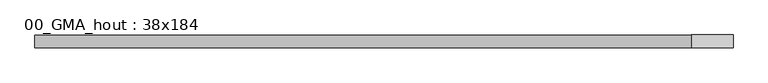
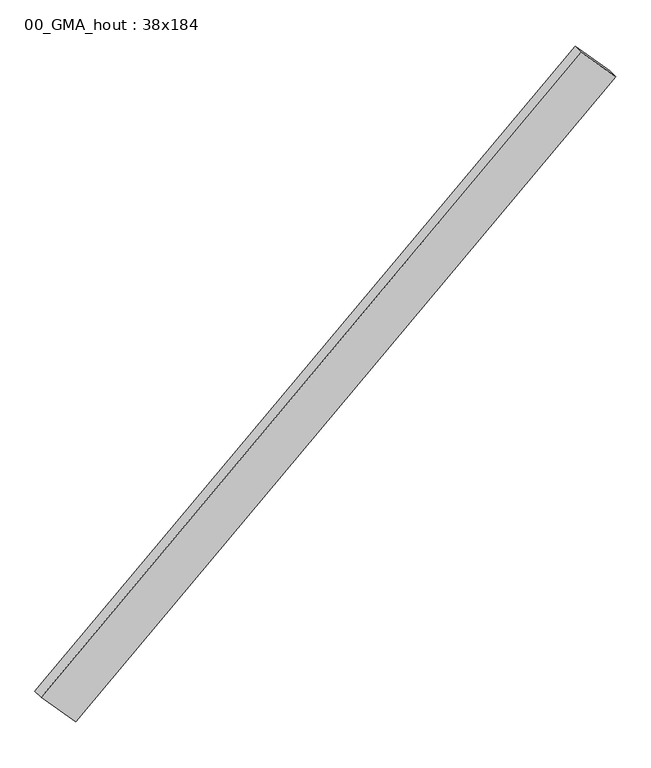
"""IFC4 building model written with IfcOpenShell, lengths in millimetres: proxy geometry, 00_GMA_hout : 38x184."""

from ifc_helpers import new_model, si_unit, frame, origin, place, context, project, spatial, polyline, outline, extrude, source, transform, mapped, element, save


def proxy_00_gma_hout_38x184_71ec18f3(model_context):
    return source(origin(), model_context, "Body", "SweptSolid", [
        extrude(outline(polyline([(-19.0, 0.0), (19.0, 0.0), (19.0, -2617.0000001), (-19.0, -2617.0000001), (-19.0, 0.0)])), frame((-400.2270235, 19.0, -613.6855812), z_axis=(-0.6735788377822399, 0.0, 0.7391153829355245), x_axis=(0.0, 1.0, 0.0)), (0.0, 0.0, 1.0), 184.0),
    ])


if __name__ == "__main__":
    model = new_model("IFC4")
    model_context = context("Model", 3, world=origin())
    ifc_project = project(units=[si_unit("LENGTHUNIT", "METRE", prefix="MILLI")], contexts=[model_context])
    site = spatial("IfcSite", under=ifc_project)
    building = spatial("IfcBuilding", under=site)
    placement = place(None, origin())
    proxy_00_gma_hout_38x184_shape = proxy_00_gma_hout_38x184_71ec18f3(model_context)
    element("IfcBuildingElementProxy", 1, Name="00_GMA_hout : 38x184", ObjectType="00_GMA_hout : 38x184", at=placement, inside=building, context=model_context, shape_type="MappedRepresentation", body=[
        mapped(proxy_00_gma_hout_38x184_shape, transform((0.0, 0.0, 0.0), x_axis=(1.0, 0.0, 0.0), y_axis=(0.0, 1.0, 0.0), z_axis=(0.0, 0.0, 1.0))),
    ])
    save(model, "model.ifc")

# Revit data of these elements
# Type "00_GMA_hout : 38x184"
#   lengte [instance default] = 1198.641 mm
#   h = 184 mm
#   b = 38 mm
#   materiaal = 00_hout_vuren_generiek
#   PositionProfile [instance default] = 00_GMP_rectangle : TopLeft
#   Default Elevation = 0
# Element 1 (IfcBuildingElementProxy, "00_GMA_hout : 38x184")
#   lengte = 2617 mm
#   Materials on its faces: "00_hout_vuren_generiek"
# Materials
#   "00_hout_vuren_generiek": class "Wood", colour RGB 255 128 0, transparency 0, Manufacturer = "RevitGG", URL = "www.revitgg.nl", Description = "Hout, vuren, generiek", Cost = 0
